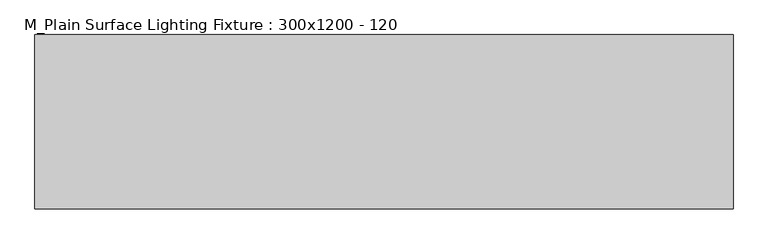
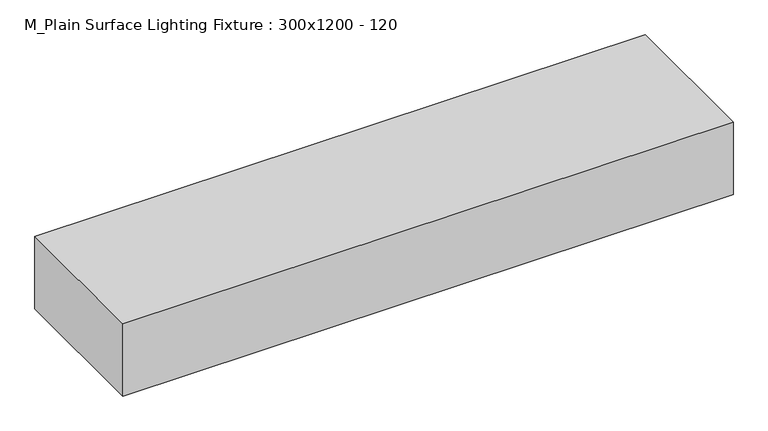
"""IFC4 building model written with IfcOpenShell, lengths in millimetres: light fixture geometry, M_Plain Surface Lighting Fixture : 300x1200 - 120."""

from ifc_helpers import new_model, si_unit, origin, origin_with_axes, place, context, project, spatial, polyline, outline, extrude, source, transform, mapped, element, save


def m_plain_surface_lighting_fixture_300x1200_120_3314c5aa(model_context):
    return source(origin(), model_context, "Body", "SweptSolid", [
        extrude(outline(polyline([(261.1478646, 738.5213005), (261.1478646, 438.5213005), (-938.8521354, 438.5213005), (-938.8521354, 738.5213005), (261.1478646, 738.5213005)])), origin_with_axes(), (0.0, 0.0, 1.0), 150.0),
    ])


if __name__ == "__main__":
    model = new_model("IFC4")
    model_context = context("Model", 3, world=origin())
    ifc_project = project(units=[si_unit("LENGTHUNIT", "METRE", prefix="MILLI")], contexts=[model_context])
    site = spatial("IfcSite", under=ifc_project)
    building = spatial("IfcBuilding", under=site)
    placement = place(None, origin())
    m_plain_surface_lighting_fixture_300x1200_120_shape = m_plain_surface_lighting_fixture_300x1200_120_3314c5aa(model_context)
    element("IfcLightFixture", 1, ObjectType="M_Plain Surface Lighting Fixture : 300x1200 - 120", at=placement, inside=building, context=model_context, shape_type="MappedRepresentation", body=[
        mapped(m_plain_surface_lighting_fixture_300x1200_120_shape, transform((0.0, 0.0, 0.0), x_axis=(1.0, 0.0, 0.0), y_axis=(0.0, 1.0, 0.0), z_axis=(0.0, 0.0, 1.0))),
    ])
    save(model, "model.ifc")

# Revit data of these elements
# Type "M_Plain Surface Lighting Fixture : 300x1200 - 120"
#   Photometric Web File = "S1x42A12.ies"
#   Width 1 = 0.15 m
#   Width = 0.30 m
#   Wattage = 64 W
#   built-in parameter 1150110 = 1 (stored number, unit not read)
#   built-in parameter 1150109 = 1 (stored number, unit not read)
#   built-in parameter 1150113 = 1 (stored number, unit not read)
#   Tilt Angle = -90.00°
#   Lumens = 5800.32 lm
#   built-in parameter 1114217 = 0.88 (stored number, unit not read)
#   built-in parameter 1150115 = 1 (stored number, unit not read)
#   built-in parameter 1150105 = 461.575 (stored number, unit not read)
#   Length 1 = 0.60 m
#   Length = 1.20 m
#   built-in parameter 1150112 = 1 (stored number, unit not read)
#   built-in parameter 1150114 = 1 (stored number, unit not read)
#   built-in parameter 1150107 = 4230 (stored number, unit not read)
#   built-in parameter 1150106 = 4.61575 (stored number, unit not read)
#   Emit from Rectangle Width = 0.30 m
#   Emit from Rectangle Length = 1.20 m
#   built-in parameter 1150104 = 8.4198 (stored number, unit not read)
#   Depth = 0.15 m
#   Default Elevation = 2.00 m
#   Ballast Voltage = 120 V
#   built-in parameter 1114218 = 0.88 (stored number, unit not read)
#   built-in parameter 1150133 = 10 (stored number, unit not read)
#   Apparent Load = 64 VA
#   built-in parameter 1150134 = 8
#   built-in parameter 1150137 = 1
#   Color Filter = 16777215
#   built-in parameter 1140040 [instance default] = 1
#   Load Classification = Lighting - Dwelling Unit
#   Emit Shape Visible in Rendering = no
#   Dimming Lamp Color Temperature Shift = (empty or 0)
